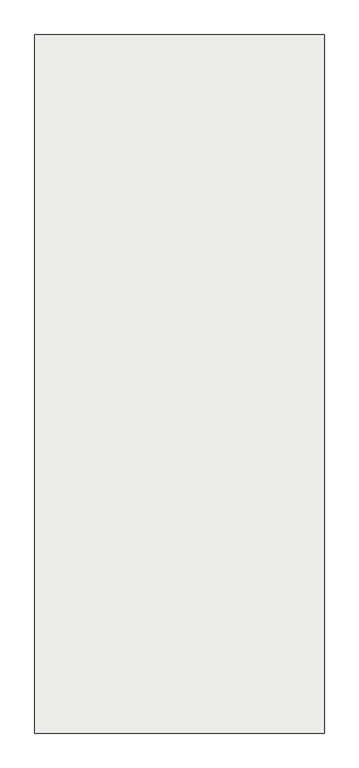
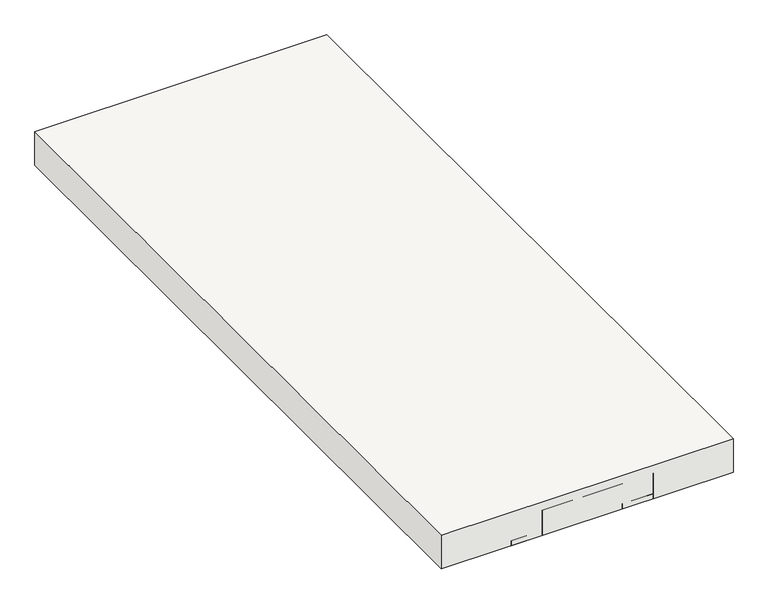
"""IFC4 building model written with IfcOpenShell, lengths in millimetres: slab geometry, Pano 4 (16 cm)."""

import ifcopenshell
import ifcopenshell.guid

model = None  # the IFC model being written
_history = None  # IfcOwnerHistory: only IFC2X3 demands one
_inside = {}  # id of a spatial element -> (the spatial element, [elements in it])
_under = {}  # id of a project, library or spatial element -> (it, [spatial elements below it])
_declared = {}  # id of a project -> (the project, [libraries it declares])
_typed = {}  # id of a type object -> (the type object, [elements of that type])
_made_of = {}  # id of a material, layer set ... -> (it, [elements and type objects made of it])


def new_model(schema):
    """Start an empty IFC model of exactly this schema.

    Asked for "IFC4X3", IfcOpenShell would pick the latest addendum, in which some entities
    have other attributes; the version numbers below select the first issue.
    IFC2X3 requires an IfcOwnerHistory on every rooted entity: one is made here for all.
    """
    global model, _history
    if schema == "IFC4X3":
        model = ifcopenshell.file(schema_version=(4, 3, 0, 0))
    else:
        model = ifcopenshell.file(schema=schema)
    _inside.clear()
    _under.clear()
    _declared.clear()
    _typed.clear()
    _made_of.clear()
    _history = None
    if model.schema == "IFC2X3":
        org = make("IfcOrganization", Name="unknown")
        user = make(
            "IfcPersonAndOrganization",
            ThePerson=make("IfcPerson", FamilyName="unknown"),
            TheOrganization=org,
        )
        app = make(
            "IfcApplication",
            ApplicationDeveloper=org,
            Version="unknown",
            ApplicationFullName="unknown",
            ApplicationIdentifier="unknown",
        )
        _history = make(
            "IfcOwnerHistory",
            OwningUser=user,
            OwningApplication=app,
            ChangeAction="ADDED",
            CreationDate=0,
        )
    return model


def make(cls, **values):
    """One entity of the class cls with the attributes given. An attribute that is None is left unset."""
    return model.create_entity(
        cls, **{name: value for name, value in values.items() if value is not None}
    )


def rooted(cls, **values):
    """An entity with a GlobalId (a new one), such as an element, a storey or a relation."""
    return make(cls, GlobalId=ifcopenshell.guid.new(), OwnerHistory=_history, **values)


def si_unit(unit_type, name, prefix=None):
    """IfcSIUnit, for example si_unit("LENGTHUNIT", "METRE", prefix="MILLI")."""
    return make("IfcSIUnit", UnitType=unit_type, Prefix=prefix, Name=name)


def assignment(units):
    """IfcUnitAssignment: the units of a project."""
    return None if units is None else make("IfcUnitAssignment", Units=units)


def point(xyz):
    """IfcCartesianPoint."""
    return None if xyz is None else make("IfcCartesianPoint", Coordinates=xyz)


def direction(xyz):
    """IfcDirection."""
    return None if xyz is None else make("IfcDirection", DirectionRatios=xyz)


def frame(location, z_axis=None, x_axis=None):
    """IfcAxis2Placement3D, a coordinate frame: its origin and axes. An axis left out is left unset."""
    return make(
        "IfcAxis2Placement3D",
        Location=point(location),
        Axis=direction(z_axis),
        RefDirection=direction(x_axis),
    )


def origin():
    """The frame at (0, 0, 0) with its axes left unset."""
    return frame((0.0, 0.0, 0.0))


def origin_with_axes():
    """The frame at (0, 0, 0) with the z axis (0, 0, 1) and the x axis (1, 0, 0) written out."""
    return frame((0.0, 0.0, 0.0), z_axis=(0.0, 0.0, 1.0), x_axis=(1.0, 0.0, 0.0))


def place(relative_to, where):
    """IfcLocalPlacement: puts the frame where relative to a parent placement (None: the world)."""
    return make(
        "IfcLocalPlacement", PlacementRelTo=relative_to, RelativePlacement=where
    )


def context(
    kind, dimensions, precision=None, world=None, true_north=None, identifier=None
):
    """IfcGeometricRepresentationContext, for example the 3D "Model" context."""
    return make(
        "IfcGeometricRepresentationContext",
        ContextIdentifier=identifier,
        ContextType=kind,
        CoordinateSpaceDimension=dimensions,
        Precision=precision,
        WorldCoordinateSystem=world,
        TrueNorth=true_north,
    )


def project(units=None, contexts=None):
    """IfcProject with its units and contexts."""
    return rooted(
        "IfcProject",
        Name="project",
        RepresentationContexts=contexts,
        UnitsInContext=assignment(units),
    )


def spatial(cls, under=None, at=None, **own):
    """A site, building, storey or space (cls), placed at a placement, below another one or the project."""
    s = rooted(cls, ObjectPlacement=at, **own)
    if under is not None:
        _under.setdefault(under.id(), (under, []))[1].append(s)
    return s


def polyline(points):
    """IfcPolyline through the points."""
    return make("IfcPolyline", Points=[point(p) for p in points])


def outline(outer, holes=None, kind="AREA"):
    """IfcArbitraryClosedProfileDef: a profile drawn as a closed curve; with holes, ...WithVoids."""
    if holes is None:
        return make("IfcArbitraryClosedProfileDef", ProfileType=kind, OuterCurve=outer)
    return make(
        "IfcArbitraryProfileDefWithVoids",
        ProfileType=kind,
        OuterCurve=outer,
        InnerCurves=holes,
    )


def extrude(swept, where, along, depth):
    """IfcExtrudedAreaSolid: the profile swept, set in the frame where, extruded along a direction by depth."""
    return make(
        "IfcExtrudedAreaSolid",
        SweptArea=swept,
        Position=where,
        ExtrudedDirection=direction(along),
        Depth=depth,
    )


def shape(context_of_items, identifier, shape_type, items):
    """IfcShapeRepresentation: the items that make up one representation, for example the "Body"."""
    return make(
        "IfcShapeRepresentation",
        ContextOfItems=context_of_items,
        RepresentationIdentifier=identifier,
        RepresentationType=shape_type,
        Items=items,
    )


def source(mapping_origin, context_of_items, identifier, shape_type, items):
    """IfcRepresentationMap: a shape defined once, which mapped items show again and again."""
    return make(
        "IfcRepresentationMap",
        MappingOrigin=mapping_origin,
        MappedRepresentation=shape(context_of_items, identifier, shape_type, items),
    )


def transform(
    local_origin,
    x_axis=None,
    y_axis=None,
    z_axis=None,
    scale=None,
    scale2=None,
    scale3=None,
    uniform=True,
):
    """IfcCartesianTransformationOperator3D, or its non-uniform kind. x_axis, y_axis, z_axis: its Axis1, 2, 3."""
    if uniform:
        return make(
            "IfcCartesianTransformationOperator3D",
            Axis1=direction(x_axis),
            Axis2=direction(y_axis),
            LocalOrigin=point(local_origin),
            Scale=scale,
            Axis3=direction(z_axis),
        )
    return make(
        "IfcCartesianTransformationOperator3DnonUniform",
        Axis1=direction(x_axis),
        Axis2=direction(y_axis),
        LocalOrigin=point(local_origin),
        Scale=scale,
        Axis3=direction(z_axis),
        Scale2=scale2,
        Scale3=scale3,
    )


def mapped(mapping_source, mapping_target):
    """IfcMappedItem: shows the shape of a source again, moved by a transform."""
    return make(
        "IfcMappedItem", MappingSource=mapping_source, MappingTarget=mapping_target
    )


def made_of(thing, what):
    """Note that an element or type object is made of a material, layer set ...; save() writes the relation."""
    if what is not None:
        _made_of.setdefault(what.id(), (what, []))[1].append(thing)
    return thing


def element(
    cls,
    number,
    at=None,
    inside=None,
    cuts=None,
    type_object=None,
    material=None,
    context=None,
    identifier="Body",
    shape_type=None,
    held_by="IfcProductDefinitionShape",
    body=None,
    shapes=None,
    **own,
):
    """One element of the class cls, such as IfcWall. Its Tag is "e" and its number.

    at: its placement. inside: the storey or other place that contains it. cuts: it is an
    opening in that element (IfcRelVoidsElement). A single representation is given by context,
    identifier, shape_type and body (its items); several are given by shapes. held_by: the class
    of the entity that holds the representations. save() writes the other relations.
    """
    e = rooted(cls, Tag="e%d" % number, ObjectPlacement=at, **own)
    if body is not None:
        shapes = [shape(context, identifier, shape_type, body)]
    if shapes is not None:
        e.Representation = make(held_by, Representations=shapes)
    if inside is not None:
        _inside.setdefault(inside.id(), (inside, []))[1].append(e)
    if cuts is not None:
        rooted(
            "IfcRelVoidsElement", RelatingBuildingElement=cuts, RelatedOpeningElement=e
        )
    if type_object is not None:
        _typed.setdefault(type_object.id(), (type_object, []))[1].append(e)
    return made_of(e, material)


def aggregate(whole, parts):
    """IfcRelAggregates: a whole, such as a stair, and the parts it consists of."""
    return rooted("IfcRelAggregates", RelatingObject=whole, RelatedObjects=parts)


def save(model, path):
    """Write the relations noted so far, then the file.

    IfcRelAggregates (storeys below a building ...), IfcRelContainedInSpatialStructure (elements
    in a storey), IfcRelDefinesByType, IfcRelAssociatesMaterial and IfcRelDeclares: one each for
    every whole, place, type object, material and project.
    """
    for whole, parts in _under.values():
        aggregate(whole, parts)
    for where, things in _inside.values():
        rooted(
            "IfcRelContainedInSpatialStructure",
            RelatedElements=things,
            RelatingStructure=where,
        )
    for kind, things in _typed.values():
        rooted("IfcRelDefinesByType", RelatedObjects=things, RelatingType=kind)
    for what, things in _made_of.values():
        rooted("IfcRelAssociatesMaterial", RelatedObjects=things, RelatingMaterial=what)
    for by, libraries in _declared.values():
        rooted("IfcRelDeclares", RelatingContext=by, RelatedDefinitions=libraries)
    model.write(path)


def slab_53e5b46f(model_context):
    return source(origin(), model_context, "Body", "SweptSolid", [
        extrude(outline(polyline([(4110.0, 1190.0), (2795.0, 1190.0), (2795.0, 4360.0), (4110.0, 4360.0), (4110.0, 1190.0)])), origin_with_axes(), (0.0, 0.0, 1.0), 160.0),
        extrude(outline(polyline([(4109.5, 3190.0), (3749.5, 3190.0), (3749.5, 3685.0), (4109.5, 3685.0), (4109.5, 3190.0)])), origin_with_axes(), (0.0, 0.0, 1.0), 120.0),
        extrude(outline(polyline([(3610.0, 2190.0), (3250.0, 2190.0), (3250.0, 2685.0), (3610.0, 2685.0), (3610.0, 2190.0)])), origin_with_axes(), (0.0, 0.0, 1.0), 120.0),
        extrude(outline(polyline([(3610.0, 2690.0), (3250.0, 2690.0), (3250.0, 3185.0), (3610.0, 3185.0), (3610.0, 2690.0)])), origin_with_axes(), (0.0, 0.0, 1.0), 120.0),
        extrude(outline(polyline([(4109.5, 2190.0), (3749.5, 2190.0), (3749.5, 2685.0), (4109.5, 2685.0), (4109.5, 2190.0)])), origin_with_axes(), (0.0, 0.0, 1.0), 120.0),
        extrude(outline(polyline([(3610.0, 3190.0), (3250.0, 3190.0), (3250.0, 3685.0), (3610.0, 3685.0), (3610.0, 3190.0)])), origin_with_axes(), (0.0, 0.0, 1.0), 120.0),
        extrude(outline(polyline([(3750.0, 1190.0), (3610.0, 1190.0), (3610.0, 4360.0), (3750.0, 4360.0), (3750.0, 1190.0)])), origin_with_axes(), (0.0, 0.0, 1.0), 24.0),
        extrude(outline(polyline([(4109.5, 3690.0), (3749.5, 3690.0), (3749.5, 4185.0), (4109.5, 4185.0), (4109.5, 3690.0)])), origin_with_axes(), (0.0, 0.0, 1.0), 120.0),
        extrude(outline(polyline([(3610.0, 1690.0), (3250.0, 1690.0), (3250.0, 2185.0), (3610.0, 2185.0), (3610.0, 1690.0)])), origin_with_axes(), (0.0, 0.0, 1.0), 120.0),
        extrude(outline(polyline([(3610.0, 4190.0), (3250.0, 4190.0), (3250.0, 4355.0), (3610.0, 4355.0), (3610.0, 4190.0)])), origin_with_axes(), (0.0, 0.0, 1.0), 120.0),
        extrude(outline(polyline([(3610.0, 3690.0), (3250.0, 3690.0), (3250.0, 4185.0), (3610.0, 4185.0), (3610.0, 3690.0)])), origin_with_axes(), (0.0, 0.0, 1.0), 120.0),
        extrude(outline(polyline([(4109.5, 2690.0), (3749.5, 2690.0), (3749.5, 3185.0), (4109.5, 3185.0), (4109.5, 2690.0)])), origin_with_axes(), (0.0, 0.0, 1.0), 120.0),
        extrude(outline(polyline([(3610.0, 1190.0), (3250.0, 1190.0), (3250.0, 1685.0), (3610.0, 1685.0), (3610.0, 1190.0)])), origin_with_axes(), (0.0, 0.0, 1.0), 120.0),
        extrude(outline(polyline([(4109.5, 1190.0), (3749.5, 1190.0), (3749.5, 1685.0), (4109.5, 1685.0), (4109.5, 1190.0)])), origin_with_axes(), (0.0, 0.0, 1.0), 120.0),
        extrude(outline(polyline([(4109.5, 1690.0), (3749.5, 1690.0), (3749.5, 2185.0), (4109.5, 2185.0), (4109.5, 1690.0)])), origin_with_axes(), (0.0, 0.0, 1.0), 120.0),
        extrude(outline(polyline([(4109.5, 4190.0), (3749.5, 4190.0), (3749.5, 4355.0), (4109.5, 4355.0), (4109.5, 4190.0)])), origin_with_axes(), (0.0, 0.0, 1.0), 120.0),
        extrude(outline(polyline([(3250.0, 1190.0), (3110.0, 1190.0), (3110.0, 4360.0), (3250.0, 4360.0), (3250.0, 1190.0)])), origin_with_axes(), (0.0, 0.0, 1.0), 24.0),
    ])


if __name__ == "__main__":
    model = new_model("IFC4")
    model_context = context("Model", 3, world=origin())
    ifc_project = project(units=[si_unit("LENGTHUNIT", "METRE", prefix="MILLI")], contexts=[model_context])
    site = spatial("IfcSite", under=ifc_project)
    building = spatial("IfcBuilding", under=site)
    placement = place(None, origin())
    slab_shape = slab_53e5b46f(model_context)
    element("IfcSlab", 1, ObjectType="Pano 4 (16 cm)", at=placement, inside=building, context=model_context, shape_type="MappedRepresentation", body=[
        mapped(slab_shape, transform((0.0, 0.0, 0.0), x_axis=(1.0, 0.0, 0.0), y_axis=(0.0, 1.0, 0.0), z_axis=(0.0, 0.0, 1.0))),
    ])
    save(model, "model.ifc")

# Revit data of these elements
# Element 1 (IfcSlab, "Pano 4 (16 cm)")
#   Materials on its faces: "Molde de poliestireno", "Concreto armado", "RGB 168-169-158"
# Materials
#   "Molde de poliestireno": class "Não atribuído", colour RGB 255 255 255, transparency 0
#   "Concreto armado": class "Não atribuído", colour RGB 168 169 158, transparency 0
#   "RGB 168-169-158": class "Não atribuído", colour RGB 168 169 158, transparency 0
